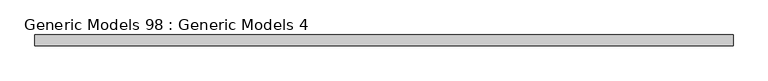
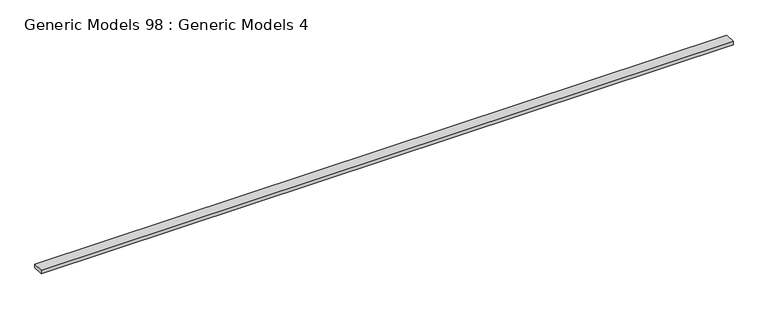
"""IFC4 building model written with IfcOpenShell, lengths in millimetres: proxy geometry, Generic Models 98 : Generic Models 4."""

from ifc_helpers import new_model, si_unit, frame, origin, place, context, project, spatial, polyline, outline, extrude, source, transform, mapped, element, save


def generic_models_98_generic_models_4_61633508(model_context):
    return source(origin(), model_context, "Body", "SweptSolid", [
        extrude(outline(polyline([(10612.5972015, 126821.946), (10325.6870839, 126821.946), (10325.6870839, 126926.4536609), (10612.5972015, 126920.4763668), (10612.5972015, 126821.946)])), frame((-10234.5171316, 0.0, 0.0), z_axis=(1.0, 0.0, 0.0), x_axis=(0.0, 1.0, 0.0)), (0.0, 0.0, 1.0), 18643.6),
    ])


if __name__ == "__main__":
    model = new_model("IFC4")
    model_context = context("Model", 3, world=origin())
    ifc_project = project(units=[si_unit("LENGTHUNIT", "METRE", prefix="MILLI")], contexts=[model_context])
    site = spatial("IfcSite", under=ifc_project)
    building = spatial("IfcBuilding", under=site)
    placement = place(None, origin())
    generic_models_98_generic_models_4_shape = generic_models_98_generic_models_4_61633508(model_context)
    element("IfcBuildingElementProxy", 1, Name="Generic Models 98 : Generic Models 4", ObjectType="Generic Models 98 : Generic Models 4", at=placement, inside=building, context=model_context, shape_type="MappedRepresentation", body=[
        mapped(generic_models_98_generic_models_4_shape, transform((0.0, 0.0, 0.0), x_axis=(1.0, 0.0, 0.0), y_axis=(0.0, 1.0, 0.0), z_axis=(0.0, 0.0, 1.0))),
    ])
    save(model, "model.ifc")

# Revit data of these elements
# Element 1 (IfcBuildingElementProxy, "Generic Models 98 : Generic Models 4")
#   Materials on its faces: "_TAPERED 2X BLOCKING (1% SLOPE) - SLOPED TOWARD DRAINS (SEE ROOF PLAN)"
# Materials
#   "_TAPERED 2X BLOCKING (1% SLOPE) - SLOPED TOWARD DRAINS (SEE ROOF PLAN)": class "Generic", colour RGB 177 130 114, transparency 0, Cost = 0
